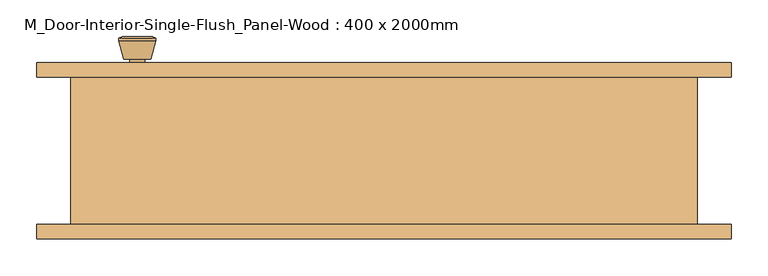
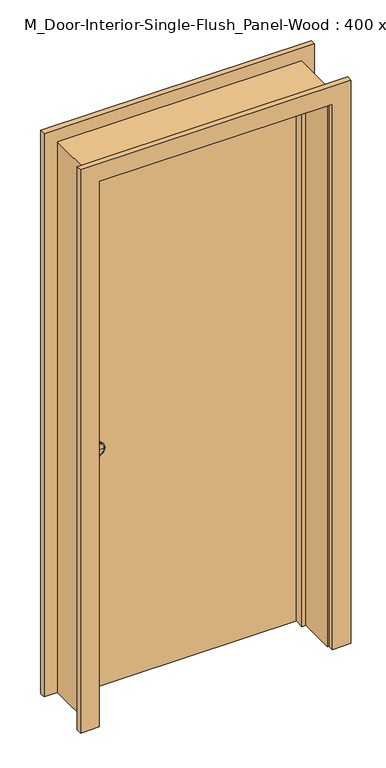
"""IFC4 building model written with IfcOpenShell, lengths in millimetres: door geometry, M_Door-Interior-Single-Flush_Panel-Wood : 400 x 2000mm."""

from ifc_helpers import new_model, si_unit, point, frame, frame_2d, origin, origin_with_axes, place, context, project, spatial, polyline, circle_curve, trimmed, segment, composite_curve, outline, extrude, faceted_brep, source, transform, mapped, element, save
from ifc_brep_helpers import plane_surface, cylinder_surface, revolved_surface, advanced_brep


def m_door_interior_single_flush_panel_wood_400_x_2000mm_76b5b41b(model_context):
    return source(origin(), model_context, "Body", "SolidModel", [
        advanced_brep(
        [(-335.0, 55.825, 914.4), (-325.0, 55.825, 914.4), (-345.0, 55.825, 914.4), (-314.5241324, 6.825, 914.4), (-335.0, 6.825, 914.4), (-355.4758676, 6.825, 914.4), (-310.0, 8.6528681, 914.4), (-360.0, 8.6528681, 914.4), (-310.0, 12.1165463, 914.4), (-360.0, 12.1165463, 914.4), (-316.363764, 36.825, 914.4), (-353.636236, 36.825, 914.4), (-325.0, 36.825, 914.4), (-345.0, 36.825, 914.4)],
        [
            (0, 1),
            (1, 2, circle_curve(frame((-335.0, 55.825, 914.4), z_axis=(0.0, 1.0, 0.0), x_axis=(-1.0, 0.0, 0.0)), 10.0)),
            (2, 0),
            (2, 1, circle_curve(frame((-335.0, 55.825, 914.4), z_axis=(0.0, 1.0, 0.0), x_axis=(-1.0, 0.0, 0.0)), 10.0)),
            (3, 4),
            (4, 5),
            (5, 3, circle_curve(frame((-335.0, 6.825, 914.4), z_axis=(0.0, -1.0, 0.0), x_axis=(-1.0, 0.0, 0.0)), 20.4758676)),
            (3, 5, circle_curve(frame((-335.0, 6.825, 914.4), z_axis=(0.0, -1.0, 0.0), x_axis=(-1.0, 0.0, 0.0)), 20.4758676)),
            (6, 3),
            (5, 7),
            (7, 6, circle_curve(frame((-335.0, 8.6528681, 914.4), z_axis=(0.0, -1.0, 0.0), x_axis=(-1.0, 0.0, 0.0)), 25.0)),
            (6, 7, circle_curve(frame((-335.0, 8.6528681, 914.4), z_axis=(0.0, -1.0, 0.0), x_axis=(-1.0, 0.0, 0.0)), 25.0)),
            (8, 6),
            (7, 9),
            (9, 8, circle_curve(frame((-335.0, 12.1165463, 914.4), z_axis=(0.0, -1.0, 0.0), x_axis=(-1.0, 0.0, 0.0)), 25.0)),
            (8, 9, circle_curve(frame((-335.0, 12.1165463, 914.4), z_axis=(0.0, -1.0, 0.0), x_axis=(-1.0, 0.0, 0.0)), 25.0)),
            (10, 8),
            (9, 11),
            (11, 10, circle_curve(frame((-335.0, 36.825, 914.4), z_axis=(0.0, -1.0, 0.0), x_axis=(-1.0, 0.0, 0.0)), 18.636236)),
            (10, 11, circle_curve(frame((-335.0, 36.825, 914.4), z_axis=(0.0, -1.0, 0.0), x_axis=(-1.0, 0.0, 0.0)), 18.636236)),
            (12, 10),
            (11, 13),
            (13, 12, circle_curve(frame((-335.0, 36.825, 914.4), z_axis=(0.0, -1.0, 0.0), x_axis=(-1.0, 0.0, 0.0)), 10.0)),
            (12, 13, circle_curve(frame((-335.0, 36.825, 914.4), z_axis=(0.0, -1.0, 0.0), x_axis=(-1.0, 0.0, 0.0)), 10.0)),
            (1, 12),
            (13, 2),
        ],
        [
            plane_surface(frame((-335.0, 55.825, 914.4), z_axis=(0.0, 1.0, 0.0), x_axis=(-1.0, 0.0, 0.0))),
            plane_surface(frame((-335.0, 6.825, 914.4), z_axis=(0.0, -1.0, 0.0), x_axis=(-1.0, 0.0, 0.0))),
            revolved_surface(polyline([(-355.4758676, 6.825, 914.4), (-360.0, 8.6528681, 914.4)]), (-335.0, 55.825, 914.4), (0.0, 1.0, 0.0)),
            cylinder_surface(frame((-335.0, 55.825, 914.4), z_axis=(0.0, 1.0, 0.0), x_axis=(-1.0, 0.0, 0.0)), 25.0),
            revolved_surface(polyline([(-360.0, 12.1165463, 914.4), (-353.636236, 36.825, 914.4)]), (-335.0, 55.825, 914.4), (0.0, 1.0, 0.0)),
            plane_surface(frame((-335.0, 36.825, 914.4), z_axis=(0.0, 1.0, 0.0), x_axis=(-1.0, 0.0, 0.0))),
            cylinder_surface(frame((-335.0, 55.825, 914.4), z_axis=(0.0, 1.0, 0.0), x_axis=(-1.0, 0.0, 0.0)), 10.0),
        ],
        [
            (0, [[1, 2, 3]]),
            (0, [[-3, 4, -1]]),
            (1, [[5, 6, 7]]),
            (1, [[-6, -5, 8]]),
            (2, [[9, -7, 10, 11]]),
            (2, [[-10, -8, -9, 12]]),
            (3, [[13, -11, 14, 15]]),
            (3, [[-14, -12, -13, 16]]),
            (4, [[17, -15, 18, 19]]),
            (4, [[-18, -16, -17, 20]]),
            (5, [[21, -19, 22, 23]]),
            (5, [[-22, -20, -21, 24]]),
            (6, [[25, -23, 26, -2]]),
            (6, [[-26, -24, -25, -4]]),
        ],
    ),
        extrude(outline(composite_curve([segment(trimmed(circle_curve(frame_2d((914.4, -335.0)), 30.0), [point((914.4, -365.0))], [point((914.4, -305.0))], False, "CARTESIAN"), True, "CONTINUOUS"), segment(trimmed(circle_curve(frame_2d((914.4, -335.0)), 30.0), [point((914.4, -305.0))], [point((914.4, -365.0))], False, "CARTESIAN"), True, "CONTINUOUS")], self_intersect=False)), frame((0.0, 55.825, 0.0), z_axis=(0.0, 1.0, 0.0), x_axis=(0.0, 0.0, 1.0)), (0.0, 0.0, 1.0), 6.0),
        advanced_brep(
        [(-335.0, 102.825, 914.4), (-345.0, 102.825, 914.4), (-325.0, 102.825, 914.4), (-314.5241324, 151.825, 914.4), (-355.4758676, 151.825, 914.4), (-335.0, 151.825, 914.4), (-310.0, 149.9971319, 914.4), (-360.0, 149.9971319, 914.4), (-310.0, 146.5334537, 914.4), (-360.0, 146.5334537, 914.4), (-316.363764, 121.825, 914.4), (-353.636236, 121.825, 914.4), (-325.0, 121.825, 914.4), (-345.0, 121.825, 914.4)],
        [
            (0, 1),
            (1, 2, circle_curve(frame((-335.0, 102.825, 914.4), z_axis=(0.0, -1.0, 0.0), x_axis=(-1.0, 0.0, 0.0)), 10.0)),
            (2, 0),
            (2, 1, circle_curve(frame((-335.0, 102.825, 914.4), z_axis=(0.0, -1.0, 0.0), x_axis=(-1.0, 0.0, 0.0)), 10.0)),
            (3, 4, circle_curve(frame((-335.0, 151.825, 914.4), z_axis=(0.0, 1.0, 0.0), x_axis=(-1.0, 0.0, 0.0)), 20.4758676)),
            (4, 5),
            (5, 3),
            (4, 3, circle_curve(frame((-335.0, 151.825, 914.4), z_axis=(0.0, 1.0, 0.0), x_axis=(-1.0, 0.0, 0.0)), 20.4758676)),
            (6, 7, circle_curve(frame((-335.0, 149.9971319, 914.4), z_axis=(0.0, 1.0, 0.0), x_axis=(-1.0, 0.0, 0.0)), 25.0)),
            (7, 4),
            (3, 6),
            (7, 6, circle_curve(frame((-335.0, 149.9971319, 914.4), z_axis=(0.0, 1.0, 0.0), x_axis=(-1.0, 0.0, 0.0)), 25.0)),
            (8, 9, circle_curve(frame((-335.0, 146.5334537, 914.4), z_axis=(0.0, 1.0, 0.0), x_axis=(-1.0, 0.0, 0.0)), 25.0)),
            (9, 7),
            (6, 8),
            (9, 8, circle_curve(frame((-335.0, 146.5334537, 914.4), z_axis=(0.0, 1.0, 0.0), x_axis=(-1.0, 0.0, 0.0)), 25.0)),
            (10, 11, circle_curve(frame((-335.0, 121.825, 914.4), z_axis=(0.0, 1.0, 0.0), x_axis=(-1.0, 0.0, 0.0)), 18.636236)),
            (11, 9),
            (8, 10),
            (11, 10, circle_curve(frame((-335.0, 121.825, 914.4), z_axis=(0.0, 1.0, 0.0), x_axis=(-1.0, 0.0, 0.0)), 18.636236)),
            (12, 13, circle_curve(frame((-335.0, 121.825, 914.4), z_axis=(0.0, 1.0, 0.0), x_axis=(-1.0, 0.0, 0.0)), 10.0)),
            (13, 11),
            (10, 12),
            (13, 12, circle_curve(frame((-335.0, 121.825, 914.4), z_axis=(0.0, 1.0, 0.0), x_axis=(-1.0, 0.0, 0.0)), 10.0)),
            (1, 13),
            (12, 2),
        ],
        [
            plane_surface(frame((-335.0, 102.825, 914.4), z_axis=(0.0, -1.0, 0.0), x_axis=(-1.0, 0.0, 0.0))),
            plane_surface(frame((-335.0, 151.825, 914.4), z_axis=(0.0, 1.0, 0.0), x_axis=(-1.0, 0.0, 0.0))),
            revolved_surface(polyline([(-355.4758676, 151.825, 914.4), (-360.0, 149.9971319, 914.4)]), (-335.0, 102.825, 914.4), (0.0, -1.0, 0.0)),
            cylinder_surface(frame((-335.0, 102.825, 914.4), z_axis=(0.0, -1.0, 0.0), x_axis=(-1.0, 0.0, 0.0)), 25.0),
            revolved_surface(polyline([(-360.0, 146.5334537, 914.4), (-353.636236, 121.825, 914.4)]), (-335.0, 102.825, 914.4), (0.0, -1.0, 0.0)),
            plane_surface(frame((-335.0, 121.825, 914.4), z_axis=(0.0, -1.0, 0.0), x_axis=(-1.0, 0.0, 0.0))),
            cylinder_surface(frame((-335.0, 102.825, 914.4), z_axis=(0.0, -1.0, 0.0), x_axis=(-1.0, 0.0, 0.0)), 10.0),
        ],
        [
            (0, [[1, 2, 3]]),
            (0, [[-3, 4, -1]]),
            (1, [[5, 6, 7]]),
            (1, [[8, -7, -6]]),
            (2, [[9, 10, -5, 11]]),
            (2, [[12, -11, -8, -10]]),
            (3, [[13, 14, -9, 15]]),
            (3, [[16, -15, -12, -14]]),
            (4, [[17, 18, -13, 19]]),
            (4, [[20, -19, -16, -18]]),
            (5, [[21, 22, -17, 23]]),
            (5, [[24, -23, -20, -22]]),
            (6, [[-2, 25, -21, 26]]),
            (6, [[-4, -26, -24, -25]]),
        ],
    ),
        extrude(outline(composite_curve([segment(trimmed(circle_curve(frame_2d((914.4, -335.0)), 30.0), [point((914.4, -365.0))], [point((914.4, -305.0))], False, "CARTESIAN"), True, "CONTINUOUS"), segment(trimmed(circle_curve(frame_2d((914.4, -335.0)), 30.0), [point((914.4, -305.0))], [point((914.4, -365.0))], False, "CARTESIAN"), True, "CONTINUOUS")], self_intersect=False)), frame((0.0, 96.825, 0.0), z_axis=(0.0, 1.0, 0.0), x_axis=(0.0, 0.0, 1.0)), (0.0, 0.0, 1.0), 6.0),
        extrude(outline(polyline([(400.0, 61.825), (-400.0, 61.825), (-400.0, 96.825), (400.0, 96.825), (400.0, 61.825)])), origin_with_axes(), (0.0, 0.0, 1.0), 2000.0),
        faceted_brep([(425.0, 96.825, 0.0), (425.0, -103.175, 0.0), (400.0, -103.175, 0.0), (400.0, 26.9, 0.0), (387.3, 26.9, 0.0), (387.3, 61.825, 0.0), (400.0, 61.825, 0.0), (400.0, 96.825, 0.0), (425.0, 96.825, 2025.0), (425.0, -103.175, 2025.0), (-425.0, -103.175, 2025.0), (-425.0, -103.175, 0.0), (-400.0, -103.175, 0.0), (-400.0, -103.175, 2000.0), (400.0, -103.175, 2000.0), (400.0, 26.9, 2000.0), (-400.0, 26.9, 2000.0), (-400.0, 26.9, 0.0), (-387.3, 26.9, 0.0), (-387.3, 26.9, 1987.3), (387.3, 26.9, 1987.3), (387.3, 61.825, 1987.3), (-387.3, 61.825, 1987.3), (-387.3, 61.825, 0.0), (-400.0, 61.825, 0.0), (-400.0, 61.825, 2000.0), (400.0, 61.825, 2000.0), (400.0, 96.825, 2000.0), (-400.0, 96.825, 2000.0), (-400.0, 96.825, 0.0), (-425.0, 96.825, 0.0), (-425.0, 96.825, 2025.0)], [[[0, 1, 2, 3, 4, 5, 6, 7]], [[1, 0, 8, 9]], [[2, 1, 9, 10, 11, 12, 13, 14]], [[3, 2, 14, 15]], [[4, 3, 15, 16, 17, 18, 19, 20]], [[5, 4, 20, 21]], [[6, 5, 21, 22, 23, 24, 25, 26]], [[7, 6, 26, 27]], [[0, 7, 27, 28, 29, 30, 31, 8]], [[9, 8, 31, 10]], [[15, 14, 13, 16]], [[21, 20, 19, 22]], [[27, 26, 25, 28]], [[30, 29, 24, 23, 18, 17, 12, 11]], [[10, 31, 30, 11]], [[16, 13, 12, 17]], [[22, 19, 18, 23]], [[28, 25, 24, 29]]]),
        extrude(outline(polyline([(0.0, 406.35), (0.0, 471.35), (2071.35, 471.35), (2071.35, -471.35), (0.0, -471.35), (0.0, -406.35), (2006.35, -406.35), (2006.35, 406.35), (0.0, 406.35)])), frame((0.0, -123.175, 0.0), z_axis=(0.0, 1.0, 0.0), x_axis=(0.0, 0.0, 1.0)), (0.0, 0.0, 1.0), 20.0),
        extrude(outline(polyline([(0.0, 406.35), (0.0, 471.35), (2071.35, 471.35), (2071.35, -471.35), (0.0, -471.35), (0.0, -406.35), (2006.35, -406.35), (2006.35, 406.35), (0.0, 406.35)])), frame((0.0, 96.825, 0.0), z_axis=(0.0, 1.0, 0.0), x_axis=(0.0, 0.0, 1.0)), (0.0, 0.0, 1.0), 20.0),
    ])


if __name__ == "__main__":
    model = new_model("IFC4")
    model_context = context("Model", 3, world=origin())
    ifc_project = project(units=[si_unit("LENGTHUNIT", "METRE", prefix="MILLI")], contexts=[model_context])
    site = spatial("IfcSite", under=ifc_project)
    building = spatial("IfcBuilding", under=site)
    placement = place(None, origin())
    m_door_interior_single_flush_panel_wood_400_x_2000mm_shape = m_door_interior_single_flush_panel_wood_400_x_2000mm_76b5b41b(model_context)
    element("IfcDoor", 1, ObjectType="M_Door-Interior-Single-Flush_Panel-Wood : 400 x 2000mm", at=placement, inside=building, context=model_context, shape_type="MappedRepresentation", body=[
        mapped(m_door_interior_single_flush_panel_wood_400_x_2000mm_shape, transform((0.0, 0.0, 0.0), x_axis=(1.0, 0.0, 0.0), y_axis=(0.0, 1.0, 0.0), z_axis=(0.0, 0.0, 1.0))),
    ])
    save(model, "model.ifc")

# Revit data of these elements
# Type "M_Door-Interior-Single-Flush_Panel-Wood : 400 x 2000mm"
#   Type Mark = "22"
#   Assembly Code = "C1020300"
#   Analytic Construction = "Wooden"
#   Thickness = 0.035 m
#   Thermal Resistance (R) = 0.455703 (m²·K)/W
#   Swing Angle [instance default] = 90.00°
#   Rough Width = 0.85 m
#   Rough Height = 2.025 m
#   Height = 2 m
#   Width = 0.8 m
#   Heat Transfer Coefficient (U) = 2.19465 W/(m²·K)
#   Trim Material = Cherry
#   Panel Material = Cherry
#   Frame Material = Cherry
#   Door Handle Material = Aluminum
#   Visual Light Transmittance = 0
#   Solar Heat Gain Coefficient = 0
#   Wall Closure = (empty or 0)
#   Function = (empty or 0)
# Element 1 (IfcDoor, "M_Door-Interior-Single-Flush_Panel-Wood : 400 x 2000mm")
#   Materials on its faces: "Cherry", "Aluminum"
# Materials
#   "Cherry": class "Wood", colour RGB 226 177 128, transparency 0, Description = "Prunus Serotina", Cost = 0
#   "Aluminum": class "Metal", colour RGB 247 247 247, transparency 0, Description = "Aluminum 6061", Cost = 0
